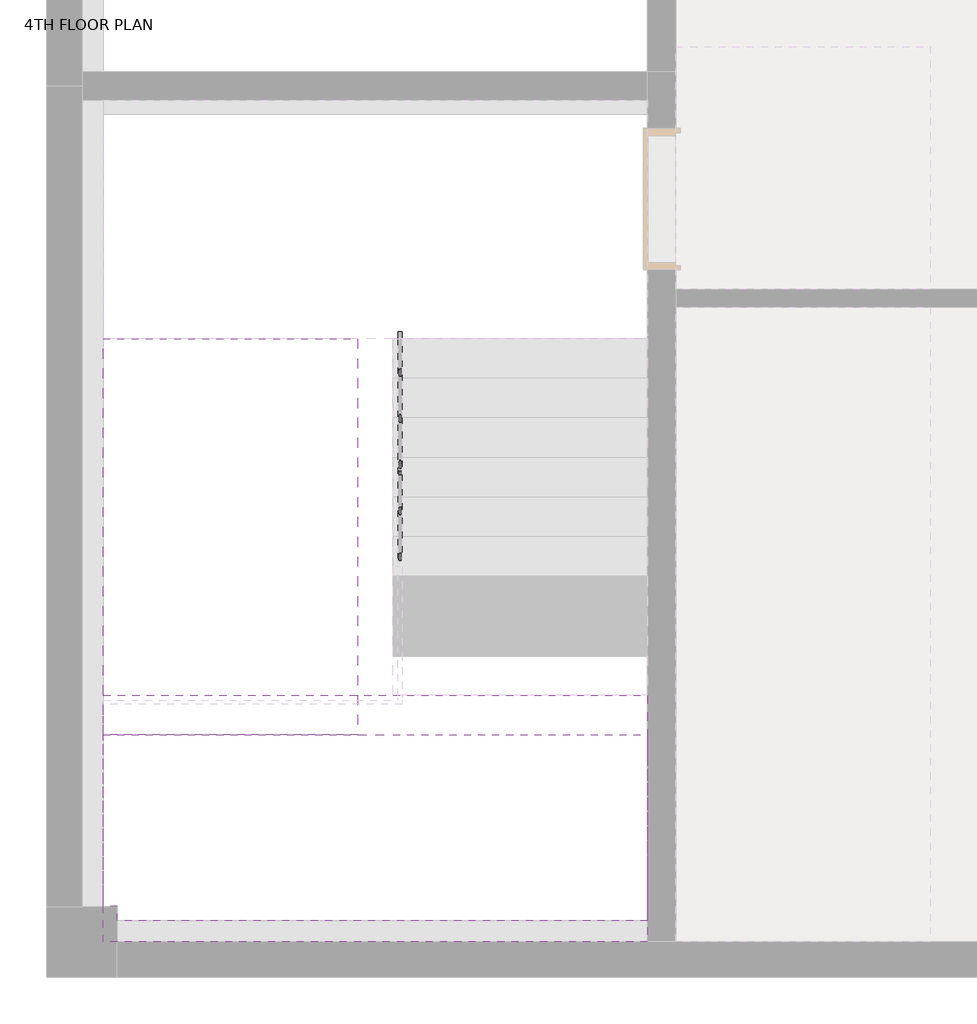
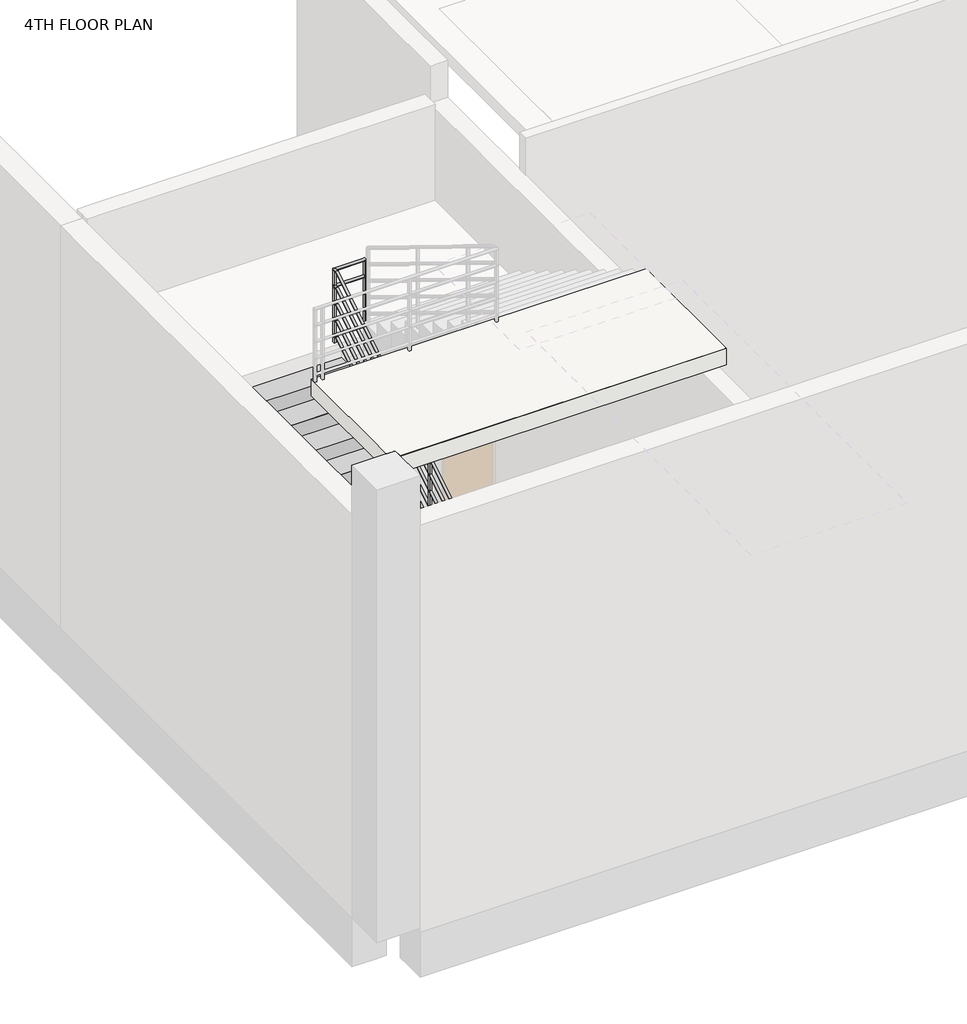
# One storey, part 5 of 6: 2 slabs, 1 railing, 1 stair flight.
"""IFC4 building model written with IfcOpenShell, lengths in millimetres."""

from ifc_helpers import new_model, si_unit, frame, origin, place, context, project, spatial, polyline, circle_curve, ellipse_curve, outline, extrude, faceted_brep, element, save
from ifc_brep_helpers import plane_surface, cylinder_surface, advanced_brep

model = new_model("IFC4")

# Units and contexts
model_context = context("Model", 3, world=origin())
ifc_project = project(units=[si_unit("LENGTHUNIT", "METRE", prefix="MILLI")], contexts=[model_context])

# Site, building, storey
site = spatial("IfcSite", under=ifc_project)
building = spatial("IfcBuilding", under=site)
storey = spatial("IfcBuildingStorey", under=building, Name="4TH FLOOR PLAN", Elevation=16100.005241)

# Railing
placement = place(None, origin())
element("IfcRailing", 1, ObjectType="900mm 배관", at=placement, inside=storey, context=model_context, shape_type="SolidModel", body=[
    advanced_brep(
    [(2135.0, 25263.5208589, 17123.587717), (2165.0, 25263.5208589, 17123.587717), (2135.0, 22409.2843108, 18875.630241), (2165.0, 22409.2843108, 18875.630241), (2135.0, 22378.5208589, 18875.630241), (2165.0, 22348.5208589, 18875.630241), (1800.0, 22378.5208589, 18875.630241), (1800.0, 22348.5208589, 18875.630241)],
    [
        (0, 1, ellipse_curve(frame((2150.0, 25263.5208589, 17123.587717), z_axis=(0.0, 1.0, 0.0), x_axis=(0.0, 0.0, -1.0)), 17.6005597, 15.0)),
        (1, 0, ellipse_curve(frame((2150.0, 25263.5208589, 17123.587717), z_axis=(0.0, 1.0, 0.0), x_axis=(0.0, 0.0, -1.0)), 17.6005597, 15.0)),
        (0, 2),
        (2, 3, ellipse_curve(frame((2150.0, 22409.2843108, 18875.630241), z_axis=(0.0, 0.9623527489128062, -0.2718035810285904), x_axis=(0.0, -0.2718035810285913, -0.9623527489128059)), 15.5868002, 15.0)),
        (3, 1),
        (3, 2, ellipse_curve(frame((2150.0, 22409.2843108, 18875.630241), z_axis=(0.0, 0.9623527489128062, -0.2718035810285904), x_axis=(0.0, -0.2718035810285913, -0.9623527489128059)), 15.5868002, 15.0)),
        (2, 4),
        (4, 5, ellipse_curve(frame((2150.0, 22363.5208589, 18875.630241), z_axis=(0.7071067811865475, 0.7071067811865475, 0.0), x_axis=(-0.7071067811865474, 0.7071067811865476, 0.0)), 21.2132034, 15.0)),
        (5, 3),
        (5, 4, ellipse_curve(frame((2150.0, 22363.5208589, 18875.630241), z_axis=(0.7071067811865475, 0.7071067811865475, 0.0), x_axis=(-0.7071067811865474, 0.7071067811865476, 0.0)), 21.2132034, 15.0)),
        (6, 7, ellipse_curve(frame((1800.0, 22363.5208589, 18875.630241), z_axis=(-0.7071067811865476, 0.0, 0.7071067811865476), x_axis=(0.7071067811865474, 0.0, 0.7071067811865478)), 21.2132034, 15.0)),
        (7, 6, ellipse_curve(frame((1800.0, 22363.5208589, 18875.630241), z_axis=(-0.7071067811865476, 0.0, 0.7071067811865476), x_axis=(0.7071067811865474, 0.0, 0.7071067811865478)), 21.2132034, 15.0)),
        (4, 6),
        (7, 5),
    ],
    [
        plane_surface(frame((2150.0, 25263.5208589, 17141.1882767), z_axis=(0.0, 1.0, 0.0), x_axis=(0.0, 0.0, -1.0))),
        cylinder_surface(frame((2150.0, 25255.6737312, 17128.4045923), z_axis=(0.0, 0.852245626680069, -0.5231418467344173), x_axis=(1.0, 0.0, 0.0)), 15.0),
        cylinder_surface(frame((2150.0, 22413.5208589, 18875.630241), z_axis=(0.0, 1.0, 0.0), x_axis=(1.0, 0.0, 0.0)), 15.0),
        plane_surface(frame((1815.0, 22363.5208589, 18890.630241), z_axis=(-0.7071067811865476, 0.0, 0.7071067811865476), x_axis=(0.7071067811865476, 0.0, 0.7071067811865476))),
        cylinder_surface(frame((2150.0, 22363.5208589, 18875.630241), z_axis=(1.0, 0.0, 0.0), x_axis=(0.0, -1.0, 0.0)), 15.0),
    ],
    [
        (0, [[1, 2]]),
        (1, [[-1, 3, 4, 5]]),
        (1, [[-2, -5, 6, -3]]),
        (2, [[-4, 7, 8, 9]]),
        (2, [[-6, -9, 10, -7]]),
        (3, [[11, 12]]),
        (4, [[-8, 13, -12, 14]]),
        (4, [[-10, -14, -11, -13]]),
    ],
),
    advanced_brep(
    [(1800.0, 22378.5208589, 18875.630241), (1800.0, 22348.5208589, 18875.630241), (1800.0, 22378.5208589, 19005.8197466), (1800.0, 22348.5208589, 19022.6056874)],
    [
        (0, 1, ellipse_curve(frame((1800.0, 22363.5208589, 18875.630241), z_axis=(0.7071067811865476, 0.0, -0.7071067811865476), x_axis=(-0.7071067811865476, 0.0, -0.7071067811865474)), 21.2132034, 15.0)),
        (1, 0, ellipse_curve(frame((1800.0, 22363.5208589, 18875.630241), z_axis=(0.7071067811865476, 0.0, -0.7071067811865476), x_axis=(-0.7071067811865476, 0.0, -0.7071067811865474)), 21.2132034, 15.0)),
        (2, 3, ellipse_curve(frame((1800.0, 22363.5208589, 19014.212717), z_axis=(0.0, 0.4882919993536566, 0.8726803099458637), x_axis=(0.0, 0.8726803099458637, -0.4882919993536565)), 17.1884249, 15.0)),
        (3, 2, ellipse_curve(frame((1800.0, 22363.5208589, 19014.212717), z_axis=(0.0, 0.4882919993536566, 0.8726803099458637), x_axis=(0.0, 0.8726803099458637, -0.4882919993536565)), 17.1884249, 15.0)),
        (0, 2),
        (3, 1),
    ],
    [
        plane_surface(frame((1800.0, 22363.5208589, 18875.630241), z_axis=(0.7071067811865476, 0.0, -0.7071067811865476), x_axis=(0.7071067811865476, 0.0, 0.7071067811865476))),
        plane_surface(frame((1800.0, 22363.5208589, 19014.212717), z_axis=(0.0, 0.4882919993536566, 0.8726803099458637), x_axis=(1.0, 0.0, 0.0))),
        cylinder_surface(frame((1800.0, 22363.5208589, 18875.630241), z_axis=(0.0, 0.0, -1.0), x_axis=(0.0, -1.0, 0.0)), 15.0),
    ],
    [
        (0, [[1, 2]]),
        (1, [[3, 4]]),
        (2, [[-1, 5, -4, 6]]),
        (2, [[-2, -6, -3, -5]]),
    ],
),
    advanced_brep(
    [(1815.0, 22363.5208589, 19014.212717), (1785.0, 22363.5208589, 19014.212717), (1815.0, 25217.757407, 20766.255241), (1785.0, 25217.757407, 20766.255241), (1815.0, 25248.5208589, 20766.255241), (1785.0, 25278.5208589, 20766.255241), (2150.0, 25248.5208589, 20766.255241), (2150.0, 25278.5208589, 20766.255241)],
    [
        (0, 1, ellipse_curve(frame((1800.0, 22363.5208589, 19014.212717), z_axis=(0.0, -0.4882919993536566, -0.8726803099458637), x_axis=(0.0, -0.8726803099458635, 0.48829199935365675)), 17.1884249, 15.0)),
        (1, 0, ellipse_curve(frame((1800.0, 22363.5208589, 19014.212717), z_axis=(0.0, -0.4882919993536566, -0.8726803099458637), x_axis=(0.0, -0.8726803099458635, 0.48829199935365675)), 17.1884249, 15.0)),
        (0, 2),
        (2, 3, ellipse_curve(frame((1800.0, 25217.757407, 20766.255241), z_axis=(0.0, -0.9623527489128062, -0.2718035810285904), x_axis=(0.0, 0.2718035810285913, -0.9623527489128059)), 15.5868002, 15.0)),
        (3, 1),
        (3, 2, ellipse_curve(frame((1800.0, 25217.757407, 20766.255241), z_axis=(0.0, -0.9623527489128062, -0.2718035810285904), x_axis=(0.0, 0.2718035810285913, -0.9623527489128059)), 15.5868002, 15.0)),
        (2, 4),
        (4, 5, ellipse_curve(frame((1800.0, 25263.5208589, 20766.255241), z_axis=(-0.7071067811865475, -0.7071067811865475, 0.0), x_axis=(0.7071067811865474, -0.7071067811865476, 0.0)), 21.2132034, 15.0)),
        (5, 3),
        (5, 4, ellipse_curve(frame((1800.0, 25263.5208589, 20766.255241), z_axis=(-0.7071067811865475, -0.7071067811865475, 0.0), x_axis=(0.7071067811865474, -0.7071067811865476, 0.0)), 21.2132034, 15.0)),
        (6, 7, circle_curve(frame((2150.0, 25263.5208589, 20766.255241), z_axis=(1.0, 0.0, 0.0), x_axis=(0.0, 1.0, 0.0)), 15.0)),
        (7, 6, circle_curve(frame((2150.0, 25263.5208589, 20766.255241), z_axis=(1.0, 0.0, 0.0), x_axis=(0.0, 1.0, 0.0)), 15.0)),
        (4, 6),
        (7, 5),
    ],
    [
        plane_surface(frame((1800.0, 22348.5208589, 19022.6056874), z_axis=(0.0, -0.4882919993536566, -0.8726803099458637), x_axis=(1.0, 0.0, 0.0))),
        cylinder_surface(frame((1800.0, 22356.3679866, 19009.822003), z_axis=(0.0, -0.852245626680069, -0.5231418467344173), x_axis=(-1.0, 0.0, 0.0)), 15.0),
        cylinder_surface(frame((1800.0, 25213.5208589, 20766.255241), z_axis=(0.0, -1.0, 0.0), x_axis=(-1.0, 0.0, 0.0)), 15.0),
        plane_surface(frame((2150.0, 25263.5208589, 20781.255241), z_axis=(1.0, 0.0, 0.0), x_axis=(0.0, 1.0, 0.0))),
        cylinder_surface(frame((1800.0, 25263.5208589, 20766.255241), z_axis=(-1.0, 0.0, 0.0), x_axis=(0.0, 1.0, 0.0)), 15.0),
    ],
    [
        (0, [[1, 2]]),
        (1, [[-1, 3, 4, 5]]),
        (1, [[-2, -5, 6, -3]]),
        (2, [[-4, 7, 8, 9]]),
        (2, [[-6, -9, 10, -7]]),
        (3, [[11, 12]]),
        (4, [[-8, 13, -12, 14]]),
        (4, [[-10, -14, -11, -13]]),
    ],
),
    advanced_brep(
    [(2165.0, 25263.5208589, 16923.587717), (2135.0, 25263.5208589, 16923.587717), (2165.0, 22409.2843108, 18675.630241), (2135.0, 22409.2843108, 18675.630241), (2165.0, 22378.5208589, 18675.630241), (2135.0, 22378.5208589, 18675.630241)],
    [
        (0, 1, ellipse_curve(frame((2150.0, 25263.5208589, 16923.587717), z_axis=(0.0, 1.0, 0.0), x_axis=(0.0, 0.0, -1.0)), 17.6005597, 15.0)),
        (1, 0, ellipse_curve(frame((2150.0, 25263.5208589, 16923.587717), z_axis=(0.0, 1.0, 0.0), x_axis=(0.0, 0.0, -1.0)), 17.6005597, 15.0)),
        (0, 2),
        (2, 3, ellipse_curve(frame((2150.0, 22409.2843108, 18675.630241), z_axis=(0.0, 0.9623527489128062, -0.2718035810285904), x_axis=(0.0, -0.2718035810285913, -0.9623527489128059)), 15.5868002, 15.0)),
        (3, 1),
        (3, 2, ellipse_curve(frame((2150.0, 22409.2843108, 18675.630241), z_axis=(0.0, 0.9623527489128062, -0.2718035810285904), x_axis=(0.0, -0.2718035810285913, -0.9623527489128059)), 15.5868002, 15.0)),
        (4, 5, circle_curve(frame((2150.0, 22378.5208589, 18675.630241), z_axis=(0.0, -1.0, 0.0), x_axis=(-1.0, 0.0, 0.0)), 15.0)),
        (5, 4, circle_curve(frame((2150.0, 22378.5208589, 18675.630241), z_axis=(0.0, -1.0, 0.0), x_axis=(-1.0, 0.0, 0.0)), 15.0)),
        (2, 4),
        (5, 3),
    ],
    [
        plane_surface(frame((2150.0, 25263.5208589, 16941.1882767), z_axis=(0.0, 1.0, 0.0), x_axis=(0.0, 0.0, -1.0))),
        cylinder_surface(frame((2150.0, 25255.6737312, 16928.4045923), z_axis=(0.0, 0.852245626680069, -0.5231418467344173), x_axis=(-1.0, 0.0, 0.0)), 15.0),
        plane_surface(frame((2150.0, 22378.5208589, 18690.630241), z_axis=(0.0, -1.0, 0.0), x_axis=(0.0, 0.0, -1.0))),
        cylinder_surface(frame((2150.0, 22413.5208589, 18675.630241), z_axis=(0.0, 1.0, 0.0), x_axis=(-1.0, 0.0, 0.0)), 15.0),
    ],
    [
        (0, [[1, 2]]),
        (1, [[-1, 3, 4, 5]]),
        (1, [[-2, -5, 6, -3]]),
        (2, [[7, 8]]),
        (3, [[-4, 9, -8, 10]]),
        (3, [[-6, -10, -7, -9]]),
    ],
),
    advanced_brep(
    [(2165.0, 22348.5208589, 18675.630241), (2165.0, 22378.5208589, 18675.630241), (1815.0, 22348.5208589, 18675.630241), (1815.0, 22378.5208589, 18675.630241)],
    [
        (0, 1, circle_curve(frame((2165.0, 22363.5208589, 18675.630241), z_axis=(1.0, 0.0, 0.0), x_axis=(0.0, 1.0, 0.0)), 15.0)),
        (1, 0, circle_curve(frame((2165.0, 22363.5208589, 18675.630241), z_axis=(1.0, 0.0, 0.0), x_axis=(0.0, 1.0, 0.0)), 15.0)),
        (2, 3, circle_curve(frame((1815.0, 22363.5208589, 18675.630241), z_axis=(-1.0, 0.0, 0.0), x_axis=(0.0, 1.0, 0.0)), 15.0)),
        (3, 2, circle_curve(frame((1815.0, 22363.5208589, 18675.630241), z_axis=(-1.0, 0.0, 0.0), x_axis=(0.0, 1.0, 0.0)), 15.0)),
        (0, 2),
        (3, 1),
    ],
    [
        plane_surface(frame((2165.0, 22363.5208589, 18690.630241), z_axis=(1.0, 0.0, 0.0), x_axis=(0.0, -1.0, 0.0))),
        plane_surface(frame((1815.0, 22363.5208589, 18690.630241), z_axis=(-1.0, 0.0, 0.0), x_axis=(0.0, -1.0, 0.0))),
        cylinder_surface(frame((2165.0, 22363.5208589, 18675.630241), z_axis=(1.0, 0.0, 0.0), x_axis=(0.0, 1.0, 0.0)), 15.0),
    ],
    [
        (0, [[1, 2]]),
        (1, [[3, 4]]),
        (2, [[-1, 5, -4, 6]]),
        (2, [[-2, -6, -3, -5]]),
    ],
),
    advanced_brep(
    [(1785.0, 22348.5208589, 18805.0051277), (1815.0, 22348.5208589, 18805.0051277), (1785.0, 25217.757407, 20566.255241), (1815.0, 25217.757407, 20566.255241), (1785.0, 25248.5208589, 20566.255241), (1815.0, 25248.5208589, 20566.255241)],
    [
        (0, 1, ellipse_curve(frame((1800.0, 22348.5208589, 18805.0051277), z_axis=(0.0, -1.0, 0.0), x_axis=(0.0, 0.0, -1.0)), 17.6005597, 15.0)),
        (1, 0, ellipse_curve(frame((1800.0, 22348.5208589, 18805.0051277), z_axis=(0.0, -1.0, 0.0), x_axis=(0.0, 0.0, -1.0)), 17.6005597, 15.0)),
        (0, 2),
        (2, 3, ellipse_curve(frame((1800.0, 25217.757407, 20566.255241), z_axis=(0.0, -0.9623527489128062, -0.2718035810285904), x_axis=(0.0, 0.2718035810285913, -0.9623527489128059)), 15.5868002, 15.0)),
        (3, 1),
        (3, 2, ellipse_curve(frame((1800.0, 25217.757407, 20566.255241), z_axis=(0.0, -0.9623527489128062, -0.2718035810285904), x_axis=(0.0, 0.2718035810285913, -0.9623527489128059)), 15.5868002, 15.0)),
        (4, 5, circle_curve(frame((1800.0, 25248.5208589, 20566.255241), z_axis=(0.0, 1.0, 0.0), x_axis=(1.0, 0.0, 0.0)), 15.0)),
        (5, 4, circle_curve(frame((1800.0, 25248.5208589, 20566.255241), z_axis=(0.0, 1.0, 0.0), x_axis=(1.0, 0.0, 0.0)), 15.0)),
        (2, 4),
        (5, 3),
    ],
    [
        plane_surface(frame((1800.0, 22348.5208589, 18822.6056874), z_axis=(0.0, -1.0, 0.0), x_axis=(0.0, 0.0, 1.0))),
        cylinder_surface(frame((1800.0, 22356.3679866, 18809.822003), z_axis=(0.0, -0.852245626680069, -0.5231418467344173), x_axis=(1.0, 0.0, 0.0)), 15.0),
        plane_surface(frame((1800.0, 25248.5208589, 20581.255241), z_axis=(0.0, 1.0, 0.0), x_axis=(0.0, 0.0, 1.0))),
        cylinder_surface(frame((1800.0, 25213.5208589, 20566.255241), z_axis=(0.0, -1.0, 0.0), x_axis=(1.0, 0.0, 0.0)), 15.0),
    ],
    [
        (0, [[1, 2]]),
        (1, [[-1, 3, 4, 5]]),
        (1, [[-2, -5, 6, -3]]),
        (2, [[7, 8]]),
        (3, [[-4, 9, -8, 10]]),
        (3, [[-6, -10, -7, -9]]),
    ],
),
    advanced_brep(
    [(1785.0, 25278.5208589, 20566.255241), (1785.0, 25248.5208589, 20566.255241), (2150.0, 25278.5208589, 20566.255241), (2150.0, 25248.5208589, 20566.255241)],
    [
        (0, 1, circle_curve(frame((1785.0, 25263.5208589, 20566.255241), z_axis=(-1.0, 0.0, 0.0), x_axis=(0.0, -1.0, 0.0)), 15.0)),
        (1, 0, circle_curve(frame((1785.0, 25263.5208589, 20566.255241), z_axis=(-1.0, 0.0, 0.0), x_axis=(0.0, -1.0, 0.0)), 15.0)),
        (2, 3, circle_curve(frame((2150.0, 25263.5208589, 20566.255241), z_axis=(1.0, 0.0, 0.0), x_axis=(0.0, -1.0, 0.0)), 15.0)),
        (3, 2, circle_curve(frame((2150.0, 25263.5208589, 20566.255241), z_axis=(1.0, 0.0, 0.0), x_axis=(0.0, -1.0, 0.0)), 15.0)),
        (0, 2),
        (3, 1),
    ],
    [
        plane_surface(frame((1785.0, 25263.5208589, 20581.255241), z_axis=(-1.0, 0.0, 0.0), x_axis=(0.0, 1.0, 0.0))),
        plane_surface(frame((2150.0, 25263.5208589, 20581.255241), z_axis=(1.0, 0.0, 0.0), x_axis=(0.0, 1.0, 0.0))),
        cylinder_surface(frame((1785.0, 25263.5208589, 20566.255241), z_axis=(-1.0, 0.0, 0.0), x_axis=(0.0, -1.0, 0.0)), 15.0),
    ],
    [
        (0, [[1, 2]]),
        (1, [[3, 4]]),
        (2, [[-1, 5, -4, 6]]),
        (2, [[-2, -6, -3, -5]]),
    ],
),
    advanced_brep(
    [(2165.0, 25263.5208589, 16723.587717), (2135.0, 25263.5208589, 16723.587717), (2165.0, 22409.2843108, 18475.630241), (2135.0, 22409.2843108, 18475.630241), (2165.0, 22378.5208589, 18475.630241), (2135.0, 22378.5208589, 18475.630241)],
    [
        (0, 1, ellipse_curve(frame((2150.0, 25263.5208589, 16723.587717), z_axis=(0.0, 1.0, 0.0), x_axis=(0.0, 0.0, -1.0)), 17.6005597, 15.0)),
        (1, 0, ellipse_curve(frame((2150.0, 25263.5208589, 16723.587717), z_axis=(0.0, 1.0, 0.0), x_axis=(0.0, 0.0, -1.0)), 17.6005597, 15.0)),
        (0, 2),
        (2, 3, ellipse_curve(frame((2150.0, 22409.2843108, 18475.630241), z_axis=(0.0, 0.9623527489128062, -0.2718035810285904), x_axis=(0.0, -0.2718035810285913, -0.9623527489128059)), 15.5868002, 15.0)),
        (3, 1),
        (3, 2, ellipse_curve(frame((2150.0, 22409.2843108, 18475.630241), z_axis=(0.0, 0.9623527489128062, -0.2718035810285904), x_axis=(0.0, -0.2718035810285913, -0.9623527489128059)), 15.5868002, 15.0)),
        (4, 5, circle_curve(frame((2150.0, 22378.5208589, 18475.630241), z_axis=(0.0, -1.0, 0.0), x_axis=(-1.0, 0.0, 0.0)), 15.0)),
        (5, 4, circle_curve(frame((2150.0, 22378.5208589, 18475.630241), z_axis=(0.0, -1.0, 0.0), x_axis=(-1.0, 0.0, 0.0)), 15.0)),
        (2, 4),
        (5, 3),
    ],
    [
        plane_surface(frame((2150.0, 25263.5208589, 16741.1882767), z_axis=(0.0, 1.0, 0.0), x_axis=(0.0, 0.0, -1.0))),
        cylinder_surface(frame((2150.0, 25255.6737312, 16728.4045923), z_axis=(0.0, 0.852245626680069, -0.5231418467344173), x_axis=(-1.0, 0.0, 0.0)), 15.0),
        plane_surface(frame((2150.0, 22378.5208589, 18490.630241), z_axis=(0.0, -1.0, 0.0), x_axis=(0.0, 0.0, -1.0))),
        cylinder_surface(frame((2150.0, 22413.5208589, 18475.630241), z_axis=(0.0, 1.0, 0.0), x_axis=(-1.0, 0.0, 0.0)), 15.0),
    ],
    [
        (0, [[1, 2]]),
        (1, [[-1, 3, 4, 5]]),
        (1, [[-2, -5, 6, -3]]),
        (2, [[7, 8]]),
        (3, [[-4, 9, -8, 10]]),
        (3, [[-6, -10, -7, -9]]),
    ],
),
    advanced_brep(
    [(2165.0, 22348.5208589, 18475.630241), (2165.0, 22378.5208589, 18475.630241), (1815.0, 22348.5208589, 18475.630241), (1815.0, 22378.5208589, 18475.630241)],
    [
        (0, 1, circle_curve(frame((2165.0, 22363.5208589, 18475.630241), z_axis=(1.0, 0.0, 0.0), x_axis=(0.0, 1.0, 0.0)), 15.0)),
        (1, 0, circle_curve(frame((2165.0, 22363.5208589, 18475.630241), z_axis=(1.0, 0.0, 0.0), x_axis=(0.0, 1.0, 0.0)), 15.0)),
        (2, 3, circle_curve(frame((1815.0, 22363.5208589, 18475.630241), z_axis=(-1.0, 0.0, 0.0), x_axis=(0.0, 1.0, 0.0)), 15.0)),
        (3, 2, circle_curve(frame((1815.0, 22363.5208589, 18475.630241), z_axis=(-1.0, 0.0, 0.0), x_axis=(0.0, 1.0, 0.0)), 15.0)),
        (0, 2),
        (3, 1),
    ],
    [
        plane_surface(frame((2165.0, 22363.5208589, 18490.630241), z_axis=(1.0, 0.0, 0.0), x_axis=(0.0, -1.0, 0.0))),
        plane_surface(frame((1815.0, 22363.5208589, 18490.630241), z_axis=(-1.0, 0.0, 0.0), x_axis=(0.0, -1.0, 0.0))),
        cylinder_surface(frame((2165.0, 22363.5208589, 18475.630241), z_axis=(1.0, 0.0, 0.0), x_axis=(0.0, 1.0, 0.0)), 15.0),
    ],
    [
        (0, [[1, 2]]),
        (1, [[3, 4]]),
        (2, [[-1, 5, -4, 6]]),
        (2, [[-2, -6, -3, -5]]),
    ],
),
    advanced_brep(
    [(1785.0, 22348.5208589, 18605.0051277), (1815.0, 22348.5208589, 18605.0051277), (1785.0, 25217.757407, 20366.255241), (1815.0, 25217.757407, 20366.255241), (1785.0, 25248.5208589, 20366.255241), (1815.0, 25248.5208589, 20366.255241)],
    [
        (0, 1, ellipse_curve(frame((1800.0, 22348.5208589, 18605.0051277), z_axis=(0.0, -1.0, 0.0), x_axis=(0.0, 0.0, -1.0)), 17.6005597, 15.0)),
        (1, 0, ellipse_curve(frame((1800.0, 22348.5208589, 18605.0051277), z_axis=(0.0, -1.0, 0.0), x_axis=(0.0, 0.0, -1.0)), 17.6005597, 15.0)),
        (0, 2),
        (2, 3, ellipse_curve(frame((1800.0, 25217.757407, 20366.255241), z_axis=(0.0, -0.9623527489128062, -0.2718035810285904), x_axis=(0.0, 0.2718035810285913, -0.9623527489128059)), 15.5868002, 15.0)),
        (3, 1),
        (3, 2, ellipse_curve(frame((1800.0, 25217.757407, 20366.255241), z_axis=(0.0, -0.9623527489128062, -0.2718035810285904), x_axis=(0.0, 0.2718035810285913, -0.9623527489128059)), 15.5868002, 15.0)),
        (4, 5, circle_curve(frame((1800.0, 25248.5208589, 20366.255241), z_axis=(0.0, 1.0, 0.0), x_axis=(1.0, 0.0, 0.0)), 15.0)),
        (5, 4, circle_curve(frame((1800.0, 25248.5208589, 20366.255241), z_axis=(0.0, 1.0, 0.0), x_axis=(1.0, 0.0, 0.0)), 15.0)),
        (2, 4),
        (5, 3),
    ],
    [
        plane_surface(frame((1800.0, 22348.5208589, 18622.6056874), z_axis=(0.0, -1.0, 0.0), x_axis=(0.0, 0.0, 1.0))),
        cylinder_surface(frame((1800.0, 22356.3679866, 18609.822003), z_axis=(0.0, -0.852245626680069, -0.5231418467344173), x_axis=(1.0, 0.0, 0.0)), 15.0),
        plane_surface(frame((1800.0, 25248.5208589, 20381.255241), z_axis=(0.0, 1.0, 0.0), x_axis=(0.0, 0.0, 1.0))),
        cylinder_surface(frame((1800.0, 25213.5208589, 20366.255241), z_axis=(0.0, -1.0, 0.0), x_axis=(1.0, 0.0, 0.0)), 15.0),
    ],
    [
        (0, [[1, 2]]),
        (1, [[-1, 3, 4, 5]]),
        (1, [[-2, -5, 6, -3]]),
        (2, [[7, 8]]),
        (3, [[-4, 9, -8, 10]]),
        (3, [[-6, -10, -7, -9]]),
    ],
),
    advanced_brep(
    [(1785.0, 25278.5208589, 20366.255241), (1785.0, 25248.5208589, 20366.255241), (2150.0, 25278.5208589, 20366.255241), (2150.0, 25248.5208589, 20366.255241)],
    [
        (0, 1, circle_curve(frame((1785.0, 25263.5208589, 20366.255241), z_axis=(-1.0, 0.0, 0.0), x_axis=(0.0, -1.0, 0.0)), 15.0)),
        (1, 0, circle_curve(frame((1785.0, 25263.5208589, 20366.255241), z_axis=(-1.0, 0.0, 0.0), x_axis=(0.0, -1.0, 0.0)), 15.0)),
        (2, 3, circle_curve(frame((2150.0, 25263.5208589, 20366.255241), z_axis=(1.0, 0.0, 0.0), x_axis=(0.0, -1.0, 0.0)), 15.0)),
        (3, 2, circle_curve(frame((2150.0, 25263.5208589, 20366.255241), z_axis=(1.0, 0.0, 0.0), x_axis=(0.0, -1.0, 0.0)), 15.0)),
        (0, 2),
        (3, 1),
    ],
    [
        plane_surface(frame((1785.0, 25263.5208589, 20381.255241), z_axis=(-1.0, 0.0, 0.0), x_axis=(0.0, 1.0, 0.0))),
        plane_surface(frame((2150.0, 25263.5208589, 20381.255241), z_axis=(1.0, 0.0, 0.0), x_axis=(0.0, 1.0, 0.0))),
        cylinder_surface(frame((1785.0, 25263.5208589, 20366.255241), z_axis=(-1.0, 0.0, 0.0), x_axis=(0.0, -1.0, 0.0)), 15.0),
    ],
    [
        (0, [[1, 2]]),
        (1, [[3, 4]]),
        (2, [[-1, 5, -4, 6]]),
        (2, [[-2, -6, -3, -5]]),
    ],
),
    advanced_brep(
    [(2165.0, 25263.5208589, 16523.587717), (2135.0, 25263.5208589, 16523.587717), (2165.0, 22409.2843108, 18275.630241), (2135.0, 22409.2843108, 18275.630241), (2165.0, 22378.5208589, 18275.630241), (2135.0, 22378.5208589, 18275.630241)],
    [
        (0, 1, ellipse_curve(frame((2150.0, 25263.5208589, 16523.587717), z_axis=(0.0, 1.0, 0.0), x_axis=(0.0, 0.0, -1.0)), 17.6005597, 15.0)),
        (1, 0, ellipse_curve(frame((2150.0, 25263.5208589, 16523.587717), z_axis=(0.0, 1.0, 0.0), x_axis=(0.0, 0.0, -1.0)), 17.6005597, 15.0)),
        (0, 2),
        (2, 3, ellipse_curve(frame((2150.0, 22409.2843108, 18275.630241), z_axis=(0.0, 0.9623527489128062, -0.2718035810285904), x_axis=(0.0, -0.2718035810285913, -0.9623527489128059)), 15.5868002, 15.0)),
        (3, 1),
        (3, 2, ellipse_curve(frame((2150.0, 22409.2843108, 18275.630241), z_axis=(0.0, 0.9623527489128062, -0.2718035810285904), x_axis=(0.0, -0.2718035810285913, -0.9623527489128059)), 15.5868002, 15.0)),
        (4, 5, circle_curve(frame((2150.0, 22378.5208589, 18275.630241), z_axis=(0.0, -1.0, 0.0), x_axis=(-1.0, 0.0, 0.0)), 15.0)),
        (5, 4, circle_curve(frame((2150.0, 22378.5208589, 18275.630241), z_axis=(0.0, -1.0, 0.0), x_axis=(-1.0, 0.0, 0.0)), 15.0)),
        (2, 4),
        (5, 3),
    ],
    [
        plane_surface(frame((2150.0, 25263.5208589, 16541.1882767), z_axis=(0.0, 1.0, 0.0), x_axis=(0.0, 0.0, -1.0))),
        cylinder_surface(frame((2150.0, 25255.6737312, 16528.4045923), z_axis=(0.0, 0.852245626680069, -0.5231418467344173), x_axis=(-1.0, 0.0, 0.0)), 15.0),
        plane_surface(frame((2150.0, 22378.5208589, 18290.630241), z_axis=(0.0, -1.0, 0.0), x_axis=(0.0, 0.0, -1.0))),
        cylinder_surface(frame((2150.0, 22413.5208589, 18275.630241), z_axis=(0.0, 1.0, 0.0), x_axis=(-1.0, 0.0, 0.0)), 15.0),
    ],
    [
        (0, [[1, 2]]),
        (1, [[-1, 3, 4, 5]]),
        (1, [[-2, -5, 6, -3]]),
        (2, [[7, 8]]),
        (3, [[-4, 9, -8, 10]]),
        (3, [[-6, -10, -7, -9]]),
    ],
),
    advanced_brep(
    [(2165.0, 22348.5208589, 18275.630241), (2165.0, 22378.5208589, 18275.630241), (1815.0, 22348.5208589, 18275.630241), (1815.0, 22378.5208589, 18275.630241)],
    [
        (0, 1, circle_curve(frame((2165.0, 22363.5208589, 18275.630241), z_axis=(1.0, 0.0, 0.0), x_axis=(0.0, 1.0, 0.0)), 15.0)),
        (1, 0, circle_curve(frame((2165.0, 22363.5208589, 18275.630241), z_axis=(1.0, 0.0, 0.0), x_axis=(0.0, 1.0, 0.0)), 15.0)),
        (2, 3, circle_curve(frame((1815.0, 22363.5208589, 18275.630241), z_axis=(-1.0, 0.0, 0.0), x_axis=(0.0, 1.0, 0.0)), 15.0)),
        (3, 2, circle_curve(frame((1815.0, 22363.5208589, 18275.630241), z_axis=(-1.0, 0.0, 0.0), x_axis=(0.0, 1.0, 0.0)), 15.0)),
        (0, 2),
        (3, 1),
    ],
    [
        plane_surface(frame((2165.0, 22363.5208589, 18290.630241), z_axis=(1.0, 0.0, 0.0), x_axis=(0.0, -1.0, 0.0))),
        plane_surface(frame((1815.0, 22363.5208589, 18290.630241), z_axis=(-1.0, 0.0, 0.0), x_axis=(0.0, -1.0, 0.0))),
        cylinder_surface(frame((2165.0, 22363.5208589, 18275.630241), z_axis=(1.0, 0.0, 0.0), x_axis=(0.0, 1.0, 0.0)), 15.0),
    ],
    [
        (0, [[1, 2]]),
        (1, [[3, 4]]),
        (2, [[-1, 5, -4, 6]]),
        (2, [[-2, -6, -3, -5]]),
    ],
),
    advanced_brep(
    [(1785.0, 22348.5208589, 18405.0051277), (1815.0, 22348.5208589, 18405.0051277), (1785.0, 25217.757407, 20166.255241), (1815.0, 25217.757407, 20166.255241), (1785.0, 25248.5208589, 20166.255241), (1815.0, 25248.5208589, 20166.255241)],
    [
        (0, 1, ellipse_curve(frame((1800.0, 22348.5208589, 18405.0051277), z_axis=(0.0, -1.0, 0.0), x_axis=(0.0, 0.0, -1.0)), 17.6005597, 15.0)),
        (1, 0, ellipse_curve(frame((1800.0, 22348.5208589, 18405.0051277), z_axis=(0.0, -1.0, 0.0), x_axis=(0.0, 0.0, -1.0)), 17.6005597, 15.0)),
        (0, 2),
        (2, 3, ellipse_curve(frame((1800.0, 25217.757407, 20166.255241), z_axis=(0.0, -0.9623527489128062, -0.2718035810285904), x_axis=(0.0, 0.2718035810285913, -0.9623527489128059)), 15.5868002, 15.0)),
        (3, 1),
        (3, 2, ellipse_curve(frame((1800.0, 25217.757407, 20166.255241), z_axis=(0.0, -0.9623527489128062, -0.2718035810285904), x_axis=(0.0, 0.2718035810285913, -0.9623527489128059)), 15.5868002, 15.0)),
        (4, 5, circle_curve(frame((1800.0, 25248.5208589, 20166.255241), z_axis=(0.0, 1.0, 0.0), x_axis=(1.0, 0.0, 0.0)), 15.0)),
        (5, 4, circle_curve(frame((1800.0, 25248.5208589, 20166.255241), z_axis=(0.0, 1.0, 0.0), x_axis=(1.0, 0.0, 0.0)), 15.0)),
        (2, 4),
        (5, 3),
    ],
    [
        plane_surface(frame((1800.0, 22348.5208589, 18422.6056874), z_axis=(0.0, -1.0, 0.0), x_axis=(0.0, 0.0, 1.0))),
        cylinder_surface(frame((1800.0, 22356.3679866, 18409.822003), z_axis=(0.0, -0.852245626680069, -0.5231418467344173), x_axis=(1.0, 0.0, 0.0)), 15.0),
        plane_surface(frame((1800.0, 25248.5208589, 20181.255241), z_axis=(0.0, 1.0, 0.0), x_axis=(0.0, 0.0, 1.0))),
        cylinder_surface(frame((1800.0, 25213.5208589, 20166.255241), z_axis=(0.0, -1.0, 0.0), x_axis=(1.0, 0.0, 0.0)), 15.0),
    ],
    [
        (0, [[1, 2]]),
        (1, [[-1, 3, 4, 5]]),
        (1, [[-2, -5, 6, -3]]),
        (2, [[7, 8]]),
        (3, [[-4, 9, -8, 10]]),
        (3, [[-6, -10, -7, -9]]),
    ],
),
    advanced_brep(
    [(1785.0, 25278.5208589, 20166.255241), (1785.0, 25248.5208589, 20166.255241), (2150.0, 25278.5208589, 20166.255241), (2150.0, 25248.5208589, 20166.255241)],
    [
        (0, 1, circle_curve(frame((1785.0, 25263.5208589, 20166.255241), z_axis=(-1.0, 0.0, 0.0), x_axis=(0.0, -1.0, 0.0)), 15.0)),
        (1, 0, circle_curve(frame((1785.0, 25263.5208589, 20166.255241), z_axis=(-1.0, 0.0, 0.0), x_axis=(0.0, -1.0, 0.0)), 15.0)),
        (2, 3, circle_curve(frame((2150.0, 25263.5208589, 20166.255241), z_axis=(1.0, 0.0, 0.0), x_axis=(0.0, -1.0, 0.0)), 15.0)),
        (3, 2, circle_curve(frame((2150.0, 25263.5208589, 20166.255241), z_axis=(1.0, 0.0, 0.0), x_axis=(0.0, -1.0, 0.0)), 15.0)),
        (0, 2),
        (3, 1),
    ],
    [
        plane_surface(frame((1785.0, 25263.5208589, 20181.255241), z_axis=(-1.0, 0.0, 0.0), x_axis=(0.0, 1.0, 0.0))),
        plane_surface(frame((2150.0, 25263.5208589, 20181.255241), z_axis=(1.0, 0.0, 0.0), x_axis=(0.0, 1.0, 0.0))),
        cylinder_surface(frame((1785.0, 25263.5208589, 20166.255241), z_axis=(-1.0, 0.0, 0.0), x_axis=(0.0, -1.0, 0.0)), 15.0),
    ],
    [
        (0, [[1, 2]]),
        (1, [[3, 4]]),
        (2, [[-1, 5, -4, 6]]),
        (2, [[-2, -6, -3, -5]]),
    ],
),
    advanced_brep(
    [(2165.0, 25263.5208589, 16323.587717), (2135.0, 25263.5208589, 16323.587717), (2165.0, 22409.2843108, 18075.630241), (2135.0, 22409.2843108, 18075.630241), (2165.0, 22378.5208589, 18075.630241), (2135.0, 22378.5208589, 18075.630241)],
    [
        (0, 1, ellipse_curve(frame((2150.0, 25263.5208589, 16323.587717), z_axis=(0.0, 1.0, 0.0), x_axis=(0.0, 0.0, -1.0)), 17.6005597, 15.0)),
        (1, 0, ellipse_curve(frame((2150.0, 25263.5208589, 16323.587717), z_axis=(0.0, 1.0, 0.0), x_axis=(0.0, 0.0, -1.0)), 17.6005597, 15.0)),
        (0, 2),
        (2, 3, ellipse_curve(frame((2150.0, 22409.2843108, 18075.630241), z_axis=(0.0, 0.9623527489128062, -0.2718035810285904), x_axis=(0.0, -0.2718035810285913, -0.9623527489128059)), 15.5868002, 15.0)),
        (3, 1),
        (3, 2, ellipse_curve(frame((2150.0, 22409.2843108, 18075.630241), z_axis=(0.0, 0.9623527489128062, -0.2718035810285904), x_axis=(0.0, -0.2718035810285913, -0.9623527489128059)), 15.5868002, 15.0)),
        (4, 5, circle_curve(frame((2150.0, 22378.5208589, 18075.630241), z_axis=(0.0, -1.0, 0.0), x_axis=(-1.0, 0.0, 0.0)), 15.0)),
        (5, 4, circle_curve(frame((2150.0, 22378.5208589, 18075.630241), z_axis=(0.0, -1.0, 0.0), x_axis=(-1.0, 0.0, 0.0)), 15.0)),
        (2, 4),
        (5, 3),
    ],
    [
        plane_surface(frame((2150.0, 25263.5208589, 16341.1882767), z_axis=(0.0, 1.0, 0.0), x_axis=(0.0, 0.0, -1.0))),
        cylinder_surface(frame((2150.0, 25255.6737312, 16328.4045923), z_axis=(0.0, 0.852245626680069, -0.5231418467344173), x_axis=(-1.0, 0.0, 0.0)), 15.0),
        plane_surface(frame((2150.0, 22378.5208589, 18090.630241), z_axis=(0.0, -1.0, 0.0), x_axis=(0.0, 0.0, -1.0))),
        cylinder_surface(frame((2150.0, 22413.5208589, 18075.630241), z_axis=(0.0, 1.0, 0.0), x_axis=(-1.0, 0.0, 0.0)), 15.0),
    ],
    [
        (0, [[1, 2]]),
        (1, [[-1, 3, 4, 5]]),
        (1, [[-2, -5, 6, -3]]),
        (2, [[7, 8]]),
        (3, [[-4, 9, -8, 10]]),
        (3, [[-6, -10, -7, -9]]),
    ],
),
    advanced_brep(
    [(2165.0, 22348.5208589, 18075.630241), (2165.0, 22378.5208589, 18075.630241), (1815.0, 22348.5208589, 18075.630241), (1815.0, 22378.5208589, 18075.630241)],
    [
        (0, 1, circle_curve(frame((2165.0, 22363.5208589, 18075.630241), z_axis=(1.0, 0.0, 0.0), x_axis=(0.0, 1.0, 0.0)), 15.0)),
        (1, 0, circle_curve(frame((2165.0, 22363.5208589, 18075.630241), z_axis=(1.0, 0.0, 0.0), x_axis=(0.0, 1.0, 0.0)), 15.0)),
        (2, 3, circle_curve(frame((1815.0, 22363.5208589, 18075.630241), z_axis=(-1.0, 0.0, 0.0), x_axis=(0.0, 1.0, 0.0)), 15.0)),
        (3, 2, circle_curve(frame((1815.0, 22363.5208589, 18075.630241), z_axis=(-1.0, 0.0, 0.0), x_axis=(0.0, 1.0, 0.0)), 15.0)),
        (0, 2),
        (3, 1),
    ],
    [
        plane_surface(frame((2165.0, 22363.5208589, 18090.630241), z_axis=(1.0, 0.0, 0.0), x_axis=(0.0, -1.0, 0.0))),
        plane_surface(frame((1815.0, 22363.5208589, 18090.630241), z_axis=(-1.0, 0.0, 0.0), x_axis=(0.0, -1.0, 0.0))),
        cylinder_surface(frame((2165.0, 22363.5208589, 18075.630241), z_axis=(1.0, 0.0, 0.0), x_axis=(0.0, 1.0, 0.0)), 15.0),
    ],
    [
        (0, [[1, 2]]),
        (1, [[3, 4]]),
        (2, [[-1, 5, -4, 6]]),
        (2, [[-2, -6, -3, -5]]),
    ],
),
    advanced_brep(
    [(1785.0, 22348.5208589, 18205.0051277), (1815.0, 22348.5208589, 18205.0051277), (1785.0, 25217.757407, 19966.255241), (1815.0, 25217.757407, 19966.255241), (1785.0, 25248.5208589, 19966.255241), (1815.0, 25248.5208589, 19966.255241)],
    [
        (0, 1, ellipse_curve(frame((1800.0, 22348.5208589, 18205.0051277), z_axis=(0.0, -1.0, 0.0), x_axis=(0.0, 0.0, -1.0)), 17.6005597, 15.0)),
        (1, 0, ellipse_curve(frame((1800.0, 22348.5208589, 18205.0051277), z_axis=(0.0, -1.0, 0.0), x_axis=(0.0, 0.0, -1.0)), 17.6005597, 15.0)),
        (0, 2),
        (2, 3, ellipse_curve(frame((1800.0, 25217.757407, 19966.255241), z_axis=(0.0, -0.9623527489128062, -0.2718035810285904), x_axis=(0.0, 0.2718035810285913, -0.9623527489128059)), 15.5868002, 15.0)),
        (3, 1),
        (3, 2, ellipse_curve(frame((1800.0, 25217.757407, 19966.255241), z_axis=(0.0, -0.9623527489128062, -0.2718035810285904), x_axis=(0.0, 0.2718035810285913, -0.9623527489128059)), 15.5868002, 15.0)),
        (4, 5, circle_curve(frame((1800.0, 25248.5208589, 19966.255241), z_axis=(0.0, 1.0, 0.0), x_axis=(1.0, 0.0, 0.0)), 15.0)),
        (5, 4, circle_curve(frame((1800.0, 25248.5208589, 19966.255241), z_axis=(0.0, 1.0, 0.0), x_axis=(1.0, 0.0, 0.0)), 15.0)),
        (2, 4),
        (5, 3),
    ],
    [
        plane_surface(frame((1800.0, 22348.5208589, 18222.6056874), z_axis=(0.0, -1.0, 0.0), x_axis=(0.0, 0.0, 1.0))),
        cylinder_surface(frame((1800.0, 22356.3679866, 18209.822003), z_axis=(0.0, -0.852245626680069, -0.5231418467344173), x_axis=(1.0, 0.0, 0.0)), 15.0),
        plane_surface(frame((1800.0, 25248.5208589, 19981.255241), z_axis=(0.0, 1.0, 0.0), x_axis=(0.0, 0.0, 1.0))),
        cylinder_surface(frame((1800.0, 25213.5208589, 19966.255241), z_axis=(0.0, -1.0, 0.0), x_axis=(1.0, 0.0, 0.0)), 15.0),
    ],
    [
        (0, [[1, 2]]),
        (1, [[-1, 3, 4, 5]]),
        (1, [[-2, -5, 6, -3]]),
        (2, [[7, 8]]),
        (3, [[-4, 9, -8, 10]]),
        (3, [[-6, -10, -7, -9]]),
    ],
),
    advanced_brep(
    [(1785.0, 25278.5208589, 19966.255241), (1785.0, 25248.5208589, 19966.255241), (2150.0, 25278.5208589, 19966.255241), (2150.0, 25248.5208589, 19966.255241)],
    [
        (0, 1, circle_curve(frame((1785.0, 25263.5208589, 19966.255241), z_axis=(-1.0, 0.0, 0.0), x_axis=(0.0, -1.0, 0.0)), 15.0)),
        (1, 0, circle_curve(frame((1785.0, 25263.5208589, 19966.255241), z_axis=(-1.0, 0.0, 0.0), x_axis=(0.0, -1.0, 0.0)), 15.0)),
        (2, 3, circle_curve(frame((2150.0, 25263.5208589, 19966.255241), z_axis=(1.0, 0.0, 0.0), x_axis=(0.0, -1.0, 0.0)), 15.0)),
        (3, 2, circle_curve(frame((2150.0, 25263.5208589, 19966.255241), z_axis=(1.0, 0.0, 0.0), x_axis=(0.0, -1.0, 0.0)), 15.0)),
        (0, 2),
        (3, 1),
    ],
    [
        plane_surface(frame((1785.0, 25263.5208589, 19981.255241), z_axis=(-1.0, 0.0, 0.0), x_axis=(0.0, 1.0, 0.0))),
        plane_surface(frame((2150.0, 25263.5208589, 19981.255241), z_axis=(1.0, 0.0, 0.0), x_axis=(0.0, 1.0, 0.0))),
        cylinder_surface(frame((1785.0, 25263.5208589, 19966.255241), z_axis=(-1.0, 0.0, 0.0), x_axis=(0.0, -1.0, 0.0)), 15.0),
    ],
    [
        (0, [[1, 2]]),
        (1, [[3, 4]]),
        (2, [[-1, 5, -4, 6]]),
        (2, [[-2, -6, -3, -5]]),
    ],
),
    extrude(outline(polyline([(24351.0208589, 20216.6177377), (24376.0208589, 20231.9637199), (24376.0208589, 19193.755241), (24351.0208589, 19193.755241), (24351.0208589, 20216.6177377)])), frame((1787.5, 0.0, 0.0), z_axis=(1.0, 0.0, 0.0), x_axis=(0.0, 1.0, 0.0)), (0.0, 0.0, 1.0), 25.0),
    extrude(outline(polyline([(23351.0208589, 19602.778452), (23376.0208589, 19618.1244341), (23376.0208589, 18678.130241), (23351.0208589, 18678.130241), (23351.0208589, 19602.778452)])), frame((1787.5, 0.0, 0.0), z_axis=(1.0, 0.0, 0.0), x_axis=(0.0, 1.0, 0.0)), (0.0, 0.0, 1.0), 25.0),
    extrude(outline(polyline([(23251.0208589, 18341.3387199), (23276.0208589, 18325.9927377), (23276.0208589, 17303.130241), (23251.0208589, 17303.130241), (23251.0208589, 18341.3387199)])), frame((2137.5, 0.0, 0.0), z_axis=(1.0, 0.0, 0.0), x_axis=(0.0, 1.0, 0.0)), (0.0, 0.0, 1.0), 25.0),
    extrude(outline(polyline([(24251.0208589, 17727.4994341), (24276.0208589, 17712.153452), (24276.0208589, 16787.505241), (24251.0208589, 16787.505241), (24251.0208589, 17727.4994341)])), frame((2137.5, 0.0, 0.0), z_axis=(1.0, 0.0, 0.0), x_axis=(0.0, 1.0, 0.0)), (0.0, 0.0, 1.0), 25.0),
    extrude(outline(polyline([(2137.5, 25251.0208589), (2137.5, 25276.0208589), (2162.5, 25276.0208589), (2162.5, 25251.0208589), (2137.5, 25251.0208589)])), frame((0.0, 0.0, 19881.255241), z_axis=(0.0, 0.0, 1.0), x_axis=(1.0, 0.0, 0.0)), (0.0, 0.0, 1.0), 870.0),
    extrude(outline(polyline([(1812.5, 25251.0208589), (1787.5, 25251.0208589), (1787.5, 25276.0208589), (1812.5, 25276.0208589), (1812.5, 25251.0208589)])), frame((0.0, 0.0, 19881.255241), z_axis=(0.0, 0.0, 1.0), x_axis=(1.0, 0.0, 0.0)), (0.0, 0.0, 1.0), 870.0),
    extrude(outline(polyline([(1812.5, 22376.0208589), (1812.5, 22351.0208589), (1787.5, 22351.0208589), (1787.5, 22376.0208589), (1812.5, 22376.0208589)])), frame((0.0, 0.0, 17990.630241), z_axis=(0.0, 0.0, 1.0), x_axis=(1.0, 0.0, 0.0)), (0.0, 0.0, 1.0), 870.0),
    extrude(outline(polyline([(2137.5, 22376.0208589), (2162.5, 22376.0208589), (2162.5, 22351.0208589), (2137.5, 22351.0208589), (2137.5, 22376.0208589)])), frame((0.0, 0.0, 17990.630241), z_axis=(0.0, 0.0, 1.0), x_axis=(1.0, 0.0, 0.0)), (0.0, 0.0, 1.0), 870.0),
])

# Slabs
element("IfcSlab", 2, ObjectType="프리캐스트 콘크리트 - 200mm 두께", at=placement, inside=storey, context=model_context, shape_type="SolidModel", body=[
    faceted_brep([(3900.0, 22413.5208589, 17989.836491), (2100.0, 22413.5208589, 17989.836491), (1850.0, 22413.5208589, 17989.836491), (50.0, 22413.5208589, 17989.836491), (50.0, 22374.4317945, 17989.836491), (50.0, 20949.5208589, 17989.836491), (3900.0, 20949.5208589, 17989.836491), (3900.0, 22172.6099233, 17989.836491), (3900.0, 22413.5208589, 17817.961491), (3900.0, 22413.5208589, 17641.9558943), (2100.0, 22413.5208589, 17641.9558943), (2100.0, 22413.5208589, 17789.836491), (1850.0, 22413.5208589, 17789.836491), (1850.0, 22413.5208589, 17813.8308943), (50.0, 22413.5208589, 17813.8308943), (50.0, 22374.4317945, 17789.836491), (50.0, 20949.5208589, 17789.836491), (3900.0, 20949.5208589, 17789.836491), (3900.0, 22172.6099233, 17789.836491), (1850.0, 22374.4317945, 17789.836491), (2100.0, 22172.6099233, 17789.836491)], [[[0, 1, 2, 3, 4, 5, 6, 7]], [[1, 0, 8, 9, 10, 11]], [[2, 1, 11, 12, 13]], [[3, 14, 15, 16, 5, 4]], [[6, 5, 16, 17]], [[9, 8, 0, 7, 6, 17, 18]], [[19, 12, 11, 20, 18, 17, 16, 15]], [[12, 19, 13]], [[18, 20, 10, 9]], [[20, 11, 10]], [[19, 15, 14, 13]], [[3, 2, 13, 14]]]),
    extrude(outline(polyline([(3900.0, 22413.5208589), (3900.0, 20949.5208589), (50.0, 20949.5208589), (50.0, 22413.5208589), (1850.0, 22413.5208589), (2100.0, 22413.5208589), (3900.0, 22413.5208589)])), frame((0.0, 0.0, 17989.836491), z_axis=(0.0, 0.0, 1.0), x_axis=(1.0, 0.0, 0.0)), (0.0, 0.0, 1.0), 0.79375),
])
element("IfcSlab", 3, ObjectType="프리캐스트 콘크리트 - 200mm 두께", at=placement, inside=storey, context=model_context, shape_type="SolidModel", body=[
    faceted_brep([(3900.0, 22693.5208589, 21599.211491), (2100.0, 22693.5208589, 21599.211491), (50.0, 22693.5208589, 21599.211491), (50.0, 21199.5208589, 21599.211491), (150.0, 21199.5208589, 21599.211491), (150.0, 21099.5208589, 21599.211491), (3900.0, 21099.5208589, 21599.211491), (3900.0, 22452.6099233, 21599.211491), (3900.0, 22693.5208589, 21251.3308943), (3900.0, 22693.5208589, 21427.336491), (3900.0, 21099.5208589, 21399.211491), (3900.0, 22452.6099233, 21399.211491), (50.0, 22693.5208589, 21399.211491), (50.0, 21199.5208589, 21399.211491), (150.0, 21199.5208589, 21399.211491), (150.0, 21099.5208589, 21399.211491), (2100.0, 22452.6099233, 21399.211491), (2100.0, 22693.5208589, 21399.211491), (2100.0, 22693.5208589, 21251.3308943)], [[[0, 1, 2, 3, 4, 5, 6, 7]], [[8, 9, 0, 7, 6, 10, 11]], [[3, 2, 12, 13]], [[4, 3, 13, 14]], [[5, 4, 14, 15]], [[6, 5, 15, 10]], [[16, 11, 10, 15, 14, 13, 12, 17]], [[1, 0, 9, 8, 18, 17]], [[2, 1, 17, 12]], [[11, 16, 18, 8]], [[16, 17, 18]]]),
    extrude(outline(polyline([(3900.0, 22693.5208589), (3900.0, 21099.5208589), (150.0, 21099.5208589), (150.0, 21199.5208589), (50.0, 21199.5208589), (50.0, 22693.5208589), (2100.0, 22693.5208589), (3900.0, 22693.5208589)])), frame((0.0, 0.0, 21599.211491), z_axis=(0.0, 0.0, 1.0), x_axis=(1.0, 0.0, 0.0)), (0.0, 0.0, 1.0), 0.79375),
])

# Stair flight
element("IfcStairFlight", 4, ObjectType="1mm 디딤판", at=placement, inside=storey, context=model_context, shape_type="SolidModel", body=[
    faceted_brep([(50.0, 22693.5208589, 18161.711491), (50.0, 22413.5208589, 18161.711491), (1850.0, 22413.5208589, 18161.711491), (1850.0, 22693.5208589, 18161.711491), (50.0, 22693.5208589, 17985.7058943), (50.0, 22413.5208589, 17813.8308943), (50.0, 22413.5208589, 17989.836491), (1850.0, 22413.5208589, 17813.8308943), (1850.0, 22693.5208589, 17985.7058943), (50.0, 22973.5208589, 18333.586491), (50.0, 22693.5208589, 18333.586491), (1850.0, 22693.5208589, 18333.586491), (1850.0, 22973.5208589, 18333.586491), (50.0, 22973.5208589, 18157.5808943), (1850.0, 22973.5208589, 18157.5808943), (50.0, 23253.5208589, 18505.461491), (50.0, 22973.5208589, 18505.461491), (1850.0, 22973.5208589, 18505.461491), (1850.0, 23253.5208589, 18505.461491), (50.0, 23253.5208589, 18329.4558943), (1850.0, 23253.5208589, 18329.4558943), (50.0, 23533.5208589, 18677.336491), (50.0, 23253.5208589, 18677.336491), (1850.0, 23253.5208589, 18677.336491), (1850.0, 23533.5208589, 18677.336491), (50.0, 23533.5208589, 18501.3308943), (1850.0, 23533.5208589, 18501.3308943), (50.0, 23813.5208589, 18849.211491), (50.0, 23533.5208589, 18849.211491), (1850.0, 23533.5208589, 18849.211491), (1850.0, 23813.5208589, 18849.211491), (50.0, 23813.5208589, 18673.2058943), (1850.0, 23813.5208589, 18673.2058943), (50.0, 24093.5208589, 19021.086491), (50.0, 23813.5208589, 19021.086491), (1850.0, 23813.5208589, 19021.086491), (1850.0, 24093.5208589, 19021.086491), (50.0, 24093.5208589, 18845.0808943), (1850.0, 24093.5208589, 18845.0808943), (50.0, 24373.5208589, 19192.961491), (50.0, 24093.5208589, 19192.961491), (1850.0, 24093.5208589, 19192.961491), (1850.0, 24373.5208589, 19192.961491), (50.0, 24373.5208589, 19016.9558943), (1850.0, 24373.5208589, 19016.9558943), (50.0, 24653.5208589, 19364.836491), (50.0, 24373.5208589, 19364.836491), (1850.0, 24373.5208589, 19364.836491), (1850.0, 24653.5208589, 19364.836491), (50.0, 24653.5208589, 19188.8308943), (1850.0, 24653.5208589, 19188.8308943), (50.0, 24933.5208589, 19536.711491), (50.0, 24653.5208589, 19536.711491), (1850.0, 24653.5208589, 19536.711491), (1850.0, 24933.5208589, 19536.711491), (50.0, 24933.5208589, 19360.7058943), (1850.0, 24933.5208589, 19360.7058943), (50.0, 25213.5208589, 19708.586491), (50.0, 24933.5208589, 19708.586491), (1850.0, 24933.5208589, 19708.586491), (1850.0, 25213.5208589, 19708.586491), (50.0, 25213.5208589, 19532.5808943), (1850.0, 25213.5208589, 19532.5808943), (1850.0, 25213.5208589, 19680.461491)], [[[0, 1, 2, 3]], [[1, 0, 4, 5, 6]], [[2, 1, 6, 5, 7]], [[3, 2, 7, 8]], [[9, 10, 11, 12]], [[10, 9, 13, 4, 0]], [[11, 10, 0, 3]], [[12, 11, 3, 8, 14]], [[15, 16, 17, 18]], [[16, 15, 19, 13, 9]], [[17, 16, 9, 12]], [[18, 17, 12, 14, 20]], [[21, 22, 23, 24]], [[22, 21, 25, 19, 15]], [[23, 22, 15, 18]], [[24, 23, 18, 20, 26]], [[27, 28, 29, 30]], [[28, 27, 31, 25, 21]], [[29, 28, 21, 24]], [[30, 29, 24, 26, 32]], [[33, 34, 35, 36]], [[34, 33, 37, 31, 27]], [[35, 34, 27, 30]], [[36, 35, 30, 32, 38]], [[39, 40, 41, 42]], [[40, 39, 43, 37, 33]], [[41, 40, 33, 36]], [[42, 41, 36, 38, 44]], [[45, 46, 47, 48]], [[46, 45, 49, 43, 39]], [[47, 46, 39, 42]], [[48, 47, 42, 44, 50]], [[51, 52, 53, 54]], [[52, 51, 55, 49, 45]], [[53, 52, 45, 48]], [[54, 53, 48, 50, 56]], [[57, 58, 59, 60]], [[58, 57, 61, 55, 51]], [[59, 58, 51, 54]], [[60, 59, 54, 56, 62, 63]], [[57, 60, 63, 62, 61]], [[5, 4, 13, 19, 25, 31, 37, 43, 49, 55, 61, 62, 56, 50, 44, 38, 32, 26, 20, 14, 8, 7]]]),
    extrude(outline(polyline([(50.0, 22693.5208589), (1850.0, 22693.5208589), (1850.0, 22413.5208589), (50.0, 22413.5208589), (50.0, 22693.5208589)])), frame((0.0, 0.0, 18161.711491), z_axis=(0.0, 0.0, 1.0), x_axis=(1.0, 0.0, 0.0)), (0.0, 0.0, 1.0), 0.79375),
    extrude(outline(polyline([(50.0, 22973.5208589), (1850.0, 22973.5208589), (1850.0, 22693.5208589), (50.0, 22693.5208589), (50.0, 22973.5208589)])), frame((0.0, 0.0, 18333.586491), z_axis=(0.0, 0.0, 1.0), x_axis=(1.0, 0.0, 0.0)), (0.0, 0.0, 1.0), 0.79375),
    extrude(outline(polyline([(50.0, 23253.5208589), (1850.0, 23253.5208589), (1850.0, 22973.5208589), (50.0, 22973.5208589), (50.0, 23253.5208589)])), frame((0.0, 0.0, 18505.461491), z_axis=(0.0, 0.0, 1.0), x_axis=(1.0, 0.0, 0.0)), (0.0, 0.0, 1.0), 0.79375),
    extrude(outline(polyline([(50.0, 23533.5208589), (1850.0, 23533.5208589), (1850.0, 23253.5208589), (50.0, 23253.5208589), (50.0, 23533.5208589)])), frame((0.0, 0.0, 18677.336491), z_axis=(0.0, 0.0, 1.0), x_axis=(1.0, 0.0, 0.0)), (0.0, 0.0, 1.0), 0.79375),
    extrude(outline(polyline([(50.0, 23813.5208589), (1850.0, 23813.5208589), (1850.0, 23533.5208589), (50.0, 23533.5208589), (50.0, 23813.5208589)])), frame((0.0, 0.0, 18849.211491), z_axis=(0.0, 0.0, 1.0), x_axis=(1.0, 0.0, 0.0)), (0.0, 0.0, 1.0), 0.79375),
    extrude(outline(polyline([(50.0, 24093.5208589), (1850.0, 24093.5208589), (1850.0, 23813.5208589), (50.0, 23813.5208589), (50.0, 24093.5208589)])), frame((0.0, 0.0, 19021.086491), z_axis=(0.0, 0.0, 1.0), x_axis=(1.0, 0.0, 0.0)), (0.0, 0.0, 1.0), 0.79375),
    extrude(outline(polyline([(50.0, 24373.5208589), (1850.0, 24373.5208589), (1850.0, 24093.5208589), (50.0, 24093.5208589), (50.0, 24373.5208589)])), frame((0.0, 0.0, 19192.961491), z_axis=(0.0, 0.0, 1.0), x_axis=(1.0, 0.0, 0.0)), (0.0, 0.0, 1.0), 0.79375),
    extrude(outline(polyline([(50.0, 24653.5208589), (1850.0, 24653.5208589), (1850.0, 24373.5208589), (50.0, 24373.5208589), (50.0, 24653.5208589)])), frame((0.0, 0.0, 19364.836491), z_axis=(0.0, 0.0, 1.0), x_axis=(1.0, 0.0, 0.0)), (0.0, 0.0, 1.0), 0.79375),
    extrude(outline(polyline([(50.0, 24933.5208589), (1850.0, 24933.5208589), (1850.0, 24653.5208589), (50.0, 24653.5208589), (50.0, 24933.5208589)])), frame((0.0, 0.0, 19536.711491), z_axis=(0.0, 0.0, 1.0), x_axis=(1.0, 0.0, 0.0)), (0.0, 0.0, 1.0), 0.79375),
    extrude(outline(polyline([(50.0, 25213.5208589), (1850.0, 25213.5208589), (1850.0, 24933.5208589), (50.0, 24933.5208589), (50.0, 25213.5208589)])), frame((0.0, 0.0, 19708.586491), z_axis=(0.0, 0.0, 1.0), x_axis=(1.0, 0.0, 0.0)), (0.0, 0.0, 1.0), 0.79375),
])

save(model, "model.ifc")

# Revit data of these elements
# Type "900mm 배관"
#   built-in parameter 1008612 = 0.019685 (stored number, unit not read)
#   built-in parameter 1008611 = 0.0984252 (stored number, unit not read)
#   built-in parameter 1008609 = 3.28084 (stored number, unit not read)
#   built-in parameter 1008604 = 0.19685 (stored number, unit not read)
#   built-in parameter 1008603 = 0.164042 (stored number, unit not read)
#   Railing Height = 900 mm
#   built-in parameter 1008630 = 2
#   built-in parameter 1008610 = 1
#   built-in parameter 1008605 = 1
#   built-in parameter 1008618 = 난간동자 - 정사각형1 : 25mm
# Element 1 (IfcRailing, "900mm 배관")
#   Phase Created = New Construction
#   Materials on its faces: "Metal - Stainless Steel,Polished"
# Elements 2, 3 (IfcSlab, "프리캐스트 콘크리트 - 200mm 두께")
#   Phase Created = New Construction
#   Materials on its faces: "A03AD032-00007_Structural Concrete_25MPa-30MPa"
# Element 4 (IfcStairFlight, "1mm 디딤판")
#   Phase Created = New Construction
#   Materials on its faces: "A03AD032-00007_Structural Concrete_25MPa-30MPa"
# Materials
#   "Metal - Stainless Steel,Polished": class "Metal", colour RGB 189 187 185, transparency 0, Description = "STEEL HANDRAIL(TYP.)", Cost = 0
#   "A03AD032-00007_Structural Concrete_25MPa-30MPa": class "Concrete", colour RGB 176 176 176, transparency 0, Keynote = "09910.A1", Description = "ACRYLIC EMULSION PAINT ON\nFAIR FACED CONC.", W00) Work Master Code = "A03AD032-00007", W01) Work Master_Lv1 = "Concrete Work", W02) Work Master_Lv2 = "Superstructure Work", W03) Work Master_Spec.1 = "Structural Concrete", W04) Work Master_Spec.2 = "Cement Type-1", W05) Work Master_Spec.3 = "25MPa < F'c (Cylinder Strength) ≤ 30MPa", Cost = 0
